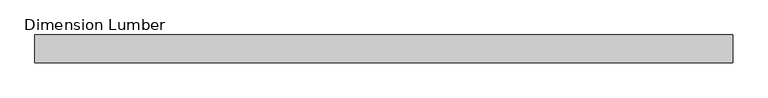
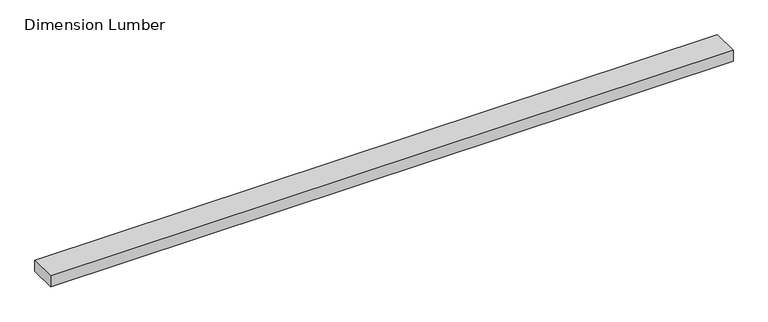
"""IFC4 building model written with IfcOpenShell, lengths in millimetres: beam geometry, Dimension Lumber : Top Supporting Lumbers."""

from ifc_helpers import new_model, si_unit, frame, origin, place, context, project, spatial, polyline, outline, extrude, source, transform, mapped, element, save


def dimension_lumber_94c0e0a3(model_context):
    return source(origin(), model_context, "Body", "SweptSolid", [
        extrude(outline(polyline([(1162.05, 44.45), (1162.05, -44.45), (-1073.15, -44.45), (-1073.15, 44.45), (1162.05, 44.45)])), frame((0.0, 0.0, -19.05), z_axis=(0.0, 0.0, 1.0), x_axis=(1.0, 0.0, 0.0)), (0.0, 0.0, 1.0), 38.1),
    ])


if __name__ == "__main__":
    model = new_model("IFC4")
    model_context = context("Model", 3, world=origin())
    ifc_project = project(units=[si_unit("LENGTHUNIT", "METRE", prefix="MILLI")], contexts=[model_context])
    site = spatial("IfcSite", under=ifc_project)
    building = spatial("IfcBuilding", under=site)
    placement = place(None, origin())
    dimension_lumber_shape = dimension_lumber_94c0e0a3(model_context)
    element("IfcBeam", 1, ObjectType="Dimension Lumber : Top Supporting Lumbers", at=placement, inside=building, context=model_context, shape_type="MappedRepresentation", body=[
        mapped(dimension_lumber_shape, transform((0.0, 0.0, 0.0), x_axis=(1.0, 0.0, 0.0), y_axis=(0.0, 1.0, 0.0), z_axis=(0.0, 0.0, 1.0))),
    ])
    save(model, "model.ifc")

# Revit data of these elements
# Type "Dimension Lumber : Top Supporting Lumbers"
#   Assembly Code = "B10"
#   A = 0.0364583 SF
#   Length [instance default] = 5' - 0"
#   b = 0' - 3 1/2"
#   d = 0' - 1 1/2"
#   Structural Material [instance default] = Softwood, Lumber
# Element 1 (IfcBeam, "Dimension Lumber : Top Supporting Lumbers")
#   Structural Material = Douglas Fir #2
#   Materials on its faces: "Douglas Fir #2"
# Materials
#   "Softwood, Lumber": class "Wood", colour RGB 223 192 134, transparency 0, Description = "Pinus Echinata", Cost = 0
#   "Douglas Fir #2": class "Wood", colour RGB 223 192 134, transparency 0, Description = "Pinus Echinata", Cost = 0
